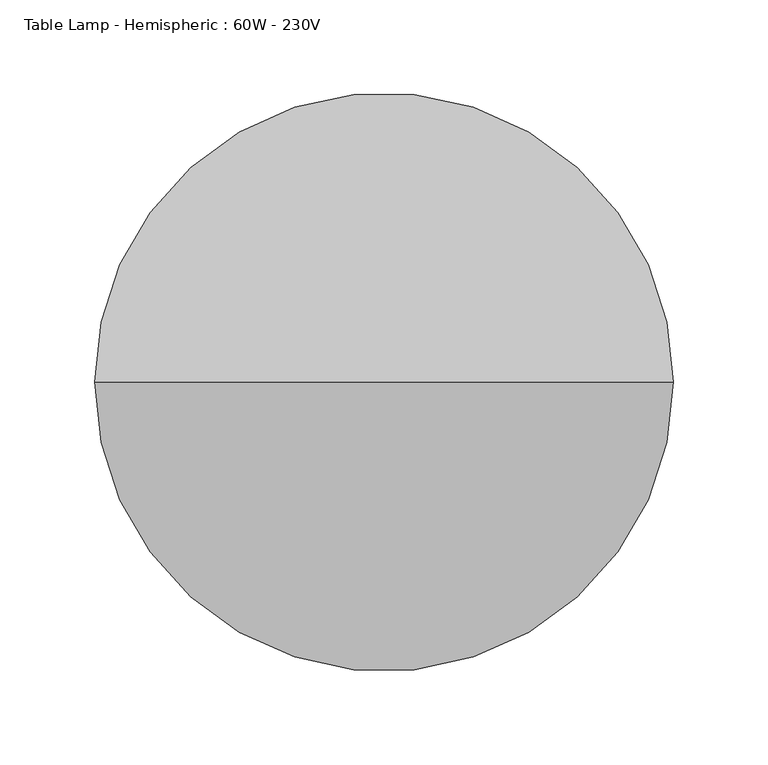
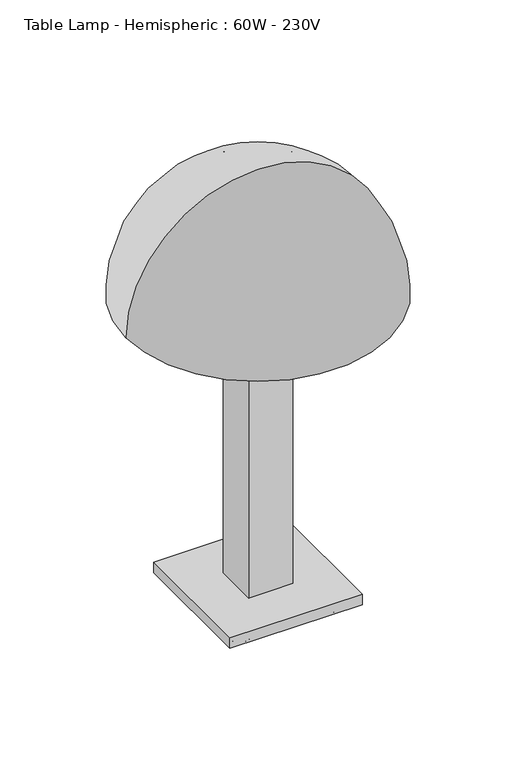
"""IFC4 building model written with IfcOpenShell, lengths in millimetres: light fixture geometry, Table Lamp - Hemispheric : 60W - 230V."""

from ifc_helpers import new_model, si_unit, point, frame, origin, origin_2d, place, context, project, spatial, polyline, circle_curve, ellipse_curve, trimmed, segment, composite_curve, outline, extrude, source, transform, mapped, element, save
from ifc_brep_helpers import plane_surface, revolved_surface, advanced_brep


def table_lamp_hemispheric_60w_230v_02721d88(model_context):
    return source(origin(), model_context, "Body", "SolidModel", [
        advanced_brep(
        [(0.0, 0.0, 524.5095504), (152.4, 0.0, 372.1095504), (-152.4, 0.0, 372.1095504), (-146.05, 0.0, 372.1095504), (146.05, 0.0, 372.1095504), (0.0, 0.0, 518.1595504)],
        [
            (0, 1, circle_curve(frame((0.0, 0.0, 372.1095504), z_axis=(0.0, 1.0, 0.0), x_axis=(1.0, 0.0, 0.0)), 152.4)),
            (1, 2, circle_curve(frame((0.0, 0.0, 372.1095504), z_axis=(0.0, 0.0, 1.0), x_axis=(1.0, 0.0, 0.0)), 152.4)),
            (2, 0, circle_curve(frame((0.0, 0.0, 372.1095504), z_axis=(0.0, 1.0, 0.0), x_axis=(-1.0, 0.0, 0.0)), 152.4)),
            (2, 1, circle_curve(frame((0.0, 0.0, 372.1095504), z_axis=(0.0, 0.0, 1.0), x_axis=(1.0, 0.0, 0.0)), 152.4)),
            (3, 4, circle_curve(frame((0.0, 0.0, 372.1095504), z_axis=(0.0, 0.0, -1.0), x_axis=(1.0, 0.0, 0.0)), 146.05)),
            (4, 5, circle_curve(frame((0.0, 0.0, 372.1095504), z_axis=(0.0, -1.0, 0.0), x_axis=(1.0, 0.0, 0.0)), 146.05)),
            (5, 3, circle_curve(frame((0.0, 0.0, 372.1095504), z_axis=(0.0, -1.0, 0.0), x_axis=(-1.0, 0.0, 0.0)), 146.05)),
            (4, 3, circle_curve(frame((0.0, 0.0, 372.1095504), z_axis=(0.0, 0.0, -1.0), x_axis=(1.0, 0.0, 0.0)), 146.05)),
            (1, 4),
            (3, 2),
        ],
        [
            revolved_surface(trimmed(ellipse_curve(frame((0.0, 0.0, 372.1095504), z_axis=(0.0, -1.0, 0.0), x_axis=(1.0, 0.0, 0.0)), 152.4, 152.4), [point((152.4, 0.0, 372.1095504))], [point((0.0, 0.0, 524.5095504))], True, "CARTESIAN"), (0.0, 0.0, 552.6321699), (0.0, 0.0, 1.0)),
            revolved_surface(trimmed(ellipse_curve(frame((0.0, 0.0, 372.1095504), z_axis=(0.0, 1.0, 0.0), x_axis=(1.0, 0.0, 0.0)), 146.05, 146.05), [point((0.0, 0.0, 518.1595504))], [point((146.05, 0.0, 372.1095504))], True, "CARTESIAN"), (0.0, 0.0, 552.6321699), (0.0, 0.0, 1.0)),
            plane_surface(frame((0.0, 0.0, 372.1095504), z_axis=(0.0, 0.0, -1.0), x_axis=(1.0, 0.0, 0.0))),
        ],
        [
            (0, [[1, 2, 3]]),
            (0, [[-3, 4, -1]]),
            (1, [[5, 6, 7]]),
            (1, [[8, -7, -6]]),
            (2, [[-2, 9, -5, 10]]),
            (2, [[-4, -10, -8, -9]]),
        ],
    ),
        extrude(outline(composite_curve([segment(trimmed(circle_curve(origin_2d(), 6.35), [point((-6.35, 0.0))], [point((6.35, 0.0))], False, "CARTESIAN"), True, "CONTINUOUS"), segment(trimmed(circle_curve(origin_2d(), 6.35), [point((6.35, 0.0))], [point((-6.35, 0.0))], False, "CARTESIAN"), True, "CONTINUOUS")], self_intersect=False)), frame((0.0, 0.0, 330.2), z_axis=(0.0, 0.0, 1.0), x_axis=(1.0, 0.0, 0.0)), (0.0, 0.0, 1.0), 63.5),
        extrude(outline(polyline([(25.4, -25.4), (-25.4, -25.4), (-25.4, 25.4), (25.4, 25.4), (25.4, -25.4)])), frame((0.0, 0.0, 25.4), z_axis=(0.0, 0.0, 1.0), x_axis=(1.0, 0.0, 0.0)), (0.0, 0.0, 1.0), 304.8),
        advanced_brep(
        [(-66.7336963, -50.8, 12.7), (-34.9836963, -50.8, 12.7), (-47.6836963, -50.8, 0.0), (-54.0336963, -50.8, 0.0), (-54.0336963, -50.8, 12.7), (-47.6836963, -50.8, 12.7)],
        [
            (0, 1, circle_curve(frame((-50.8586963, -50.8, 12.7), z_axis=(0.0, 0.0, -1.0), x_axis=(1.0, 0.0, 0.0)), 15.875)),
            (1, 2, circle_curve(frame((-47.6836963, -50.8, 12.7), z_axis=(0.0, 1.0, 0.0), x_axis=(1.0, 0.0, 0.0)), 12.7)),
            (2, 3, circle_curve(frame((-50.8586963, -50.8, 0.0), z_axis=(0.0, 0.0, 1.0), x_axis=(1.0, 0.0, 0.0)), 3.175)),
            (3, 0, circle_curve(frame((-54.0336963, -50.8, 12.7), z_axis=(0.0, 1.0, 0.0), x_axis=(-1.0, 0.0, 0.0)), 12.7)),
            (1, 0, circle_curve(frame((-50.8586963, -50.8, 12.7), z_axis=(0.0, 0.0, -1.0), x_axis=(1.0, 0.0, 0.0)), 15.875)),
            (3, 2, circle_curve(frame((-50.8586963, -50.8, 0.0), z_axis=(0.0, 0.0, 1.0), x_axis=(1.0, 0.0, 0.0)), 3.175)),
            (4, 5, circle_curve(frame((-50.8586963, -50.8, 12.7), z_axis=(0.0, 0.0, -1.0), x_axis=(1.0, 0.0, 0.0)), 3.175)),
            (5, 1),
            (0, 4),
            (5, 4, circle_curve(frame((-50.8586963, -50.8, 12.7), z_axis=(0.0, 0.0, -1.0), x_axis=(1.0, 0.0, 0.0)), 3.175)),
            (2, 5),
            (4, 3),
        ],
        [
            revolved_surface(trimmed(ellipse_curve(frame((-47.6836963, -50.8, 12.7), z_axis=(0.0, -1.0, 0.0), x_axis=(1.0, 0.0, 0.0)), 12.7, 12.7), [point((-47.6836963, -50.8, 0.0))], [point((-34.9836963, -50.8, 12.7))], True, "CARTESIAN"), (-50.8586963, -50.8, 36.0623287), (0.0, 0.0, 1.0)),
            plane_surface(frame((-50.8586963, -50.8, 12.7), z_axis=(0.0, 0.0, 1.0), x_axis=(1.0, 0.0, 0.0))),
            revolved_surface(polyline([(-47.6836963, -50.8, 12.7), (-47.6836963, -50.8, 0.0)]), (-50.8586963, -50.8, 36.0623287), (0.0, 0.0, 1.0)),
        ],
        [
            (0, [[1, 2, 3, 4]]),
            (0, [[5, -4, 6, -2]]),
            (1, [[7, 8, -1, 9]]),
            (1, [[10, -9, -5, -8]]),
            (2, [[-3, 11, -7, 12]]),
            (2, [[-6, -12, -10, -11]]),
        ],
    ),
        advanced_brep(
        [(-66.7581301, 50.8, 12.7), (-35.0081301, 50.8, 12.7), (-47.7081301, 50.8, 0.0), (-54.0581301, 50.8, 0.0), (-54.0581301, 50.8, 12.7), (-47.7081301, 50.8, 12.7)],
        [
            (0, 1, circle_curve(frame((-50.8831301, 50.8, 12.7), z_axis=(0.0, 0.0, -1.0), x_axis=(1.0, 0.0, 0.0)), 15.875)),
            (1, 2, circle_curve(frame((-47.7081301, 50.8, 12.7), z_axis=(0.0, 1.0, 0.0), x_axis=(1.0, 0.0, 0.0)), 12.7)),
            (2, 3, circle_curve(frame((-50.8831301, 50.8, 0.0), z_axis=(0.0, 0.0, 1.0), x_axis=(1.0, 0.0, 0.0)), 3.175)),
            (3, 0, circle_curve(frame((-54.0581301, 50.8, 12.7), z_axis=(0.0, 1.0, 0.0), x_axis=(-1.0, 0.0, 0.0)), 12.7)),
            (1, 0, circle_curve(frame((-50.8831301, 50.8, 12.7), z_axis=(0.0, 0.0, -1.0), x_axis=(1.0, 0.0, 0.0)), 15.875)),
            (3, 2, circle_curve(frame((-50.8831301, 50.8, 0.0), z_axis=(0.0, 0.0, 1.0), x_axis=(1.0, 0.0, 0.0)), 3.175)),
            (4, 5, circle_curve(frame((-50.8831301, 50.8, 12.7), z_axis=(0.0, 0.0, -1.0), x_axis=(1.0, 0.0, 0.0)), 3.175)),
            (5, 1),
            (0, 4),
            (5, 4, circle_curve(frame((-50.8831301, 50.8, 12.7), z_axis=(0.0, 0.0, -1.0), x_axis=(1.0, 0.0, 0.0)), 3.175)),
            (2, 5),
            (4, 3),
        ],
        [
            revolved_surface(trimmed(ellipse_curve(frame((-47.7081301, 50.8, 12.7), z_axis=(0.0, -1.0, 0.0), x_axis=(1.0, 0.0, 0.0)), 12.7, 12.7), [point((-47.7081301, 50.8, 0.0))], [point((-35.0081301, 50.8, 12.7))], True, "CARTESIAN"), (-50.8831301, 50.8, 36.0623287), (0.0, 0.0, 1.0)),
            plane_surface(frame((-50.8831301, 50.8, 12.7), z_axis=(0.0, 0.0, 1.0), x_axis=(1.0, 0.0, 0.0))),
            revolved_surface(polyline([(-47.708130100000005, 50.8, 12.7), (-47.708130100000005, 50.8, 0.0)]), (-50.8831301, 50.8, 36.0623287), (0.0, 0.0, 1.0)),
        ],
        [
            (0, [[1, 2, 3, 4]]),
            (0, [[5, -4, 6, -2]]),
            (1, [[7, 8, -1, 9]]),
            (1, [[10, -9, -5, -8]]),
            (2, [[-3, 11, -7, 12]]),
            (2, [[-6, -12, -10, -11]]),
        ],
    ),
        advanced_brep(
        [(34.9494337, -50.8, 12.7), (66.6994337, -50.8, 12.7), (53.9994337, -50.8, 0.0), (47.6494337, -50.8, 0.0), (47.6494337, -50.8, 12.7), (53.9994337, -50.8, 12.7)],
        [
            (0, 1, circle_curve(frame((50.8244337, -50.8, 12.7), z_axis=(0.0, 0.0, -1.0), x_axis=(1.0, 0.0, 0.0)), 15.875)),
            (1, 2, circle_curve(frame((53.9994337, -50.8, 12.7), z_axis=(0.0, 1.0, 0.0), x_axis=(1.0, 0.0, 0.0)), 12.7)),
            (2, 3, circle_curve(frame((50.8244337, -50.8, 0.0), z_axis=(0.0, 0.0, 1.0), x_axis=(1.0, 0.0, 0.0)), 3.175)),
            (3, 0, circle_curve(frame((47.6494337, -50.8, 12.7), z_axis=(0.0, 1.0, 0.0), x_axis=(-1.0, 0.0, 0.0)), 12.7)),
            (1, 0, circle_curve(frame((50.8244337, -50.8, 12.7), z_axis=(0.0, 0.0, -1.0), x_axis=(1.0, 0.0, 0.0)), 15.875)),
            (3, 2, circle_curve(frame((50.8244337, -50.8, 0.0), z_axis=(0.0, 0.0, 1.0), x_axis=(1.0, 0.0, 0.0)), 3.175)),
            (4, 5, circle_curve(frame((50.8244337, -50.8, 12.7), z_axis=(0.0, 0.0, -1.0), x_axis=(1.0, 0.0, 0.0)), 3.175)),
            (5, 1),
            (0, 4),
            (5, 4, circle_curve(frame((50.8244337, -50.8, 12.7), z_axis=(0.0, 0.0, -1.0), x_axis=(1.0, 0.0, 0.0)), 3.175)),
            (2, 5),
            (4, 3),
        ],
        [
            revolved_surface(trimmed(ellipse_curve(frame((53.9994337, -50.8, 12.7), z_axis=(0.0, -1.0, 0.0), x_axis=(1.0, 0.0, 0.0)), 12.7, 12.7), [point((53.9994337, -50.8, 0.0))], [point((66.6994337, -50.8, 12.7))], True, "CARTESIAN"), (50.8244337, -50.8, 36.0623287), (0.0, 0.0, 1.0)),
            plane_surface(frame((50.8244337, -50.8, 12.7), z_axis=(0.0, 0.0, 1.0), x_axis=(1.0, 0.0, 0.0))),
            revolved_surface(polyline([(53.9994337, -50.8, 12.7), (53.9994337, -50.8, 0.0)]), (50.8244337, -50.8, 36.0623287), (0.0, 0.0, 1.0)),
        ],
        [
            (0, [[1, 2, 3, 4]]),
            (0, [[5, -4, 6, -2]]),
            (1, [[7, 8, -1, 9]]),
            (1, [[10, -9, -5, -8]]),
            (2, [[-3, 11, -7, 12]]),
            (2, [[-6, -12, -10, -11]]),
        ],
    ),
        advanced_brep(
        [(34.925, 50.8, 12.7), (66.675, 50.8, 12.7), (53.975, 50.8, 0.0), (47.625, 50.8, 0.0), (47.625, 50.8, 12.7), (53.975, 50.8, 12.7)],
        [
            (0, 1, circle_curve(frame((50.8, 50.8, 12.7), z_axis=(0.0, 0.0, -1.0), x_axis=(1.0, 0.0, 0.0)), 15.875)),
            (1, 2, circle_curve(frame((53.975, 50.8, 12.7), z_axis=(0.0, 1.0, 0.0), x_axis=(1.0, 0.0, 0.0)), 12.7)),
            (2, 3, circle_curve(frame((50.8, 50.8, 0.0), z_axis=(0.0, 0.0, 1.0), x_axis=(1.0, 0.0, 0.0)), 3.175)),
            (3, 0, circle_curve(frame((47.625, 50.8, 12.7), z_axis=(0.0, 1.0, 0.0), x_axis=(-1.0, 0.0, 0.0)), 12.7)),
            (1, 0, circle_curve(frame((50.8, 50.8, 12.7), z_axis=(0.0, 0.0, -1.0), x_axis=(1.0, 0.0, 0.0)), 15.875)),
            (3, 2, circle_curve(frame((50.8, 50.8, 0.0), z_axis=(0.0, 0.0, 1.0), x_axis=(1.0, 0.0, 0.0)), 3.175)),
            (4, 5, circle_curve(frame((50.8, 50.8, 12.7), z_axis=(0.0, 0.0, -1.0), x_axis=(1.0, 0.0, 0.0)), 3.175)),
            (5, 1),
            (0, 4),
            (5, 4, circle_curve(frame((50.8, 50.8, 12.7), z_axis=(0.0, 0.0, -1.0), x_axis=(1.0, 0.0, 0.0)), 3.175)),
            (2, 5),
            (4, 3),
        ],
        [
            revolved_surface(trimmed(ellipse_curve(frame((53.975, 50.8, 12.7), z_axis=(0.0, -1.0, 0.0), x_axis=(1.0, 0.0, 0.0)), 12.7, 12.7), [point((53.975, 50.8, 0.0))], [point((66.675, 50.8, 12.7))], True, "CARTESIAN"), (50.8, 50.8, 36.0623287), (0.0, 0.0, 1.0)),
            plane_surface(frame((50.8, 50.8, 12.7), z_axis=(0.0, 0.0, 1.0), x_axis=(1.0, 0.0, 0.0))),
            revolved_surface(polyline([(53.974999999999994, 50.8, 12.7), (53.974999999999994, 50.8, 0.0)]), (50.8, 50.8, 36.0623287), (0.0, 0.0, 1.0)),
        ],
        [
            (0, [[1, 2, 3, 4]]),
            (0, [[5, -4, 6, -2]]),
            (1, [[7, 8, -1, 9]]),
            (1, [[10, -9, -5, -8]]),
            (2, [[-3, 11, -7, 12]]),
            (2, [[-6, -12, -10, -11]]),
        ],
    ),
        extrude(outline(polyline([(76.2, 76.2), (76.2, -76.2), (-76.2, -76.2), (-76.2, 76.2), (76.2, 76.2)])), frame((0.0, 0.0, 12.7), z_axis=(0.0, 0.0, 1.0), x_axis=(1.0, 0.0, 0.0)), (0.0, 0.0, 1.0), 12.7),
    ])


if __name__ == "__main__":
    model = new_model("IFC4")
    model_context = context("Model", 3, world=origin())
    ifc_project = project(units=[si_unit("LENGTHUNIT", "METRE", prefix="MILLI")], contexts=[model_context])
    site = spatial("IfcSite", under=ifc_project)
    building = spatial("IfcBuilding", under=site)
    placement = place(None, origin())
    table_lamp_hemispheric_60w_230v_shape = table_lamp_hemispheric_60w_230v_02721d88(model_context)
    element("IfcLightFixture", 1, ObjectType="Table Lamp - Hemispheric : 60W - 230V", at=placement, inside=building, context=model_context, shape_type="MappedRepresentation", body=[
        mapped(table_lamp_hemispheric_60w_230v_shape, transform((0.0, 0.0, 0.0), x_axis=(1.0, 0.0, 0.0), y_axis=(0.0, 1.0, 0.0), z_axis=(0.0, 0.0, 1.0))),
    ])
    save(model, "model.ifc")

# Revit data of these elements
# Type "Table Lamp - Hemispheric : 60W - 230V"
#   Type Mark = "Table Lamp - Hemispheric"
#   Classification.OmniClass.23.Number = "23-35 47 11"
#   Classification.OmniClass.23.Description = "Lighting Fixtures"
#   COBie.Type.CreatedBy = "info@mma.ie"
#   COBie.Type.CreatedOn = "2017-07-25T10:15:16"
#   COBie.Type.Name = "Table Lamp - Hemispheric"
#   COBie.Type.Category = "23-35 47 11 : Lighting Fixtures"
#   COBie.Type.Description = "Table Lamp - Hemispheric_60W - 230V"
#   COBie.Type.AssetType = "Movable"
#   COBie.Type.Manufacturer = ""
#   COBie.Type.ModelNumber = ""
#   Photometric Web File = "TLAE1A19.ies"
#   Keynote = "26 51 13.B"
#   Assembly Code = "D5020220"
#   Lamp = "A-19"
#   COBie.Type.ReplacementCost = 0
#   Wattage = 60 W
#   built-in parameter 1150110 = 1 (stored number, unit not read)
#   built-in parameter 1114217 = 1 (stored number, unit not read)
#   built-in parameter 1150109 = 1 (stored number, unit not read)
#   T.L. Tilt Angle = 90.00°
#   T.L. Efficacy = 14.25 lm/W
#   built-in parameter 1150113 = 1 (stored number, unit not read)
#   Tilt Angle = 90.00°
#   built-in parameter 1150115 = 1 (stored number, unit not read)
#   built-in parameter 1150105 = 68.0387 (stored number, unit not read)
#   built-in parameter 1150112 = 1 (stored number, unit not read)
#   built-in parameter 1150114 = 1 (stored number, unit not read)
#   built-in parameter 1150107 = 2800 (stored number, unit not read)
#   built-in parameter 1150106 = 0.680387 (stored number, unit not read)
#   built-in parameter 1150104 = 1.32387 (stored number, unit not read)
#   Ballast Voltage = 230 V
#   built-in parameter 1114218 = 1 (stored number, unit not read)
#   built-in parameter 1150133 = 10 (stored number, unit not read)
#   Lumens = 855 lm
#   Apparent Load = 60 VA
#   COBie.Type = yes
#   built-in parameter 1150134 = 4
#   built-in parameter 1150137 = 1
#   Color Filter = 16777215
#   Ballast Number of Poles = 1
#   T.L. Material = Wood - Birch
#   Mount Material = Metal - Chrome
#   Load Classification = Lighting - Dwelling Unit
#   Shade Material = Glass - Frosted
#   Base Material = Wood - Birch
#   Dimming Lamp Color Temperature Shift = (empty or 0)
#   Default Elevation = 0
#   Wattage Comments = ""
# Element 1 (IfcLightFixture, "Table Lamp - Hemispheric : 60W - 230V")
#   Materials on its faces: "Metal - Chrome", "Glass - Frosted", "Wood - Birch"
# Materials
#   "Wood - Birch": class "Wood", colour RGB 224 178 126, transparency 0
#   "Metal - Chrome": class "Metal", colour RGB 17 17 17, transparency 0, Comments = "Rendering appearance not upgraded "
#   "Glass - Frosted": class "Glass", colour RGB 250 244 225, transparency 0.55
